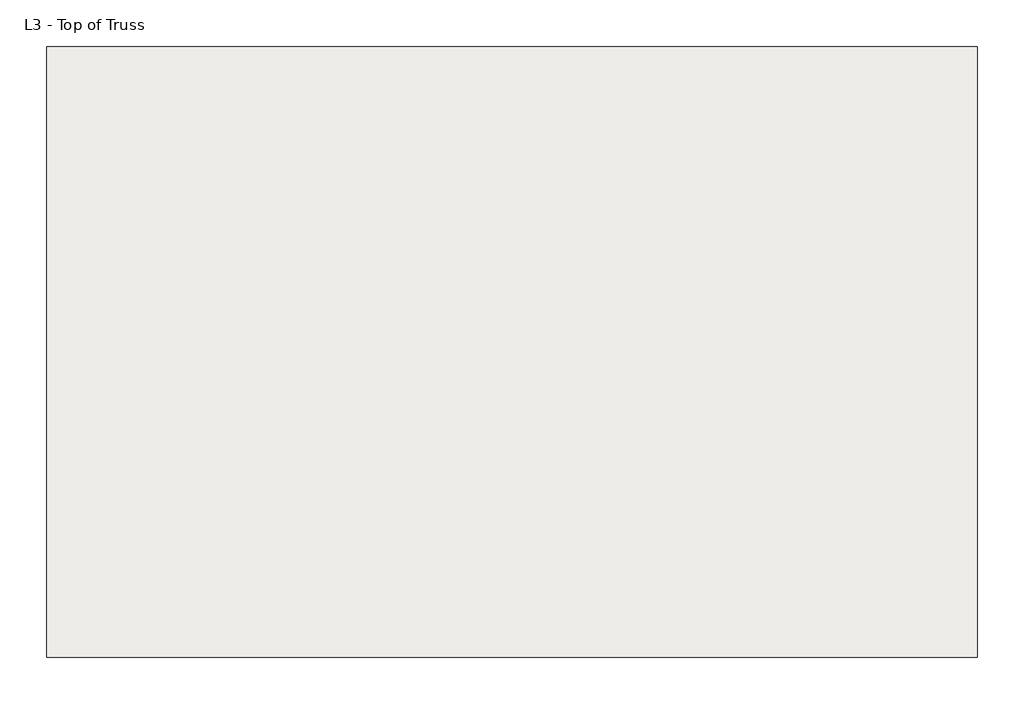
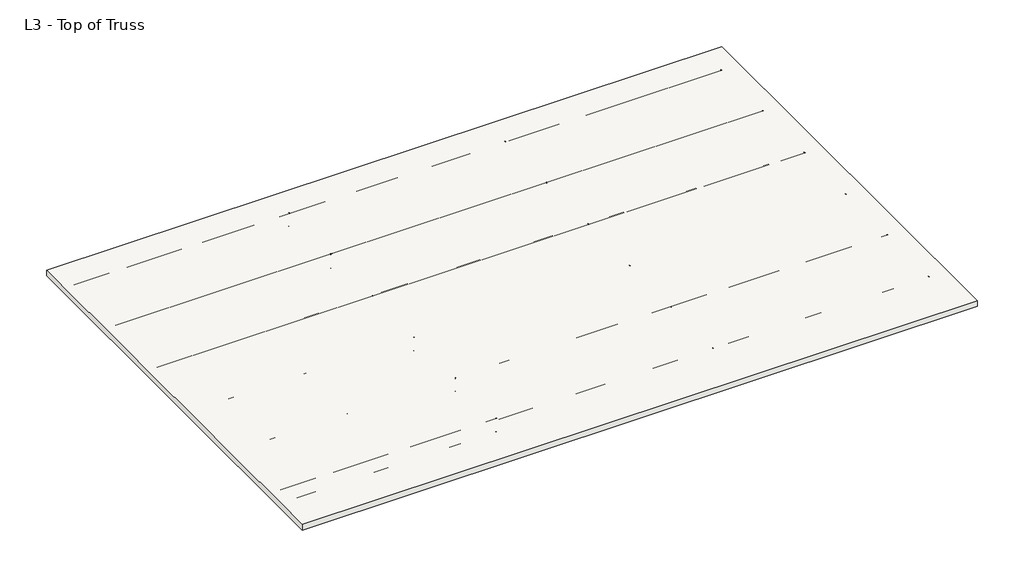
# One storey, part 1 of 2: 98 beams, 1 roof.
"""IFC4 building model written with IfcOpenShell, lengths in millimetres."""

import ifcopenshell
import ifcopenshell.guid

model = None  # the IFC model being written
_history = None  # IfcOwnerHistory: only IFC2X3 demands one
_inside = {}  # id of a spatial element -> (the spatial element, [elements in it])
_under = {}  # id of a project, library or spatial element -> (it, [spatial elements below it])
_declared = {}  # id of a project -> (the project, [libraries it declares])
_typed = {}  # id of a type object -> (the type object, [elements of that type])
_made_of = {}  # id of a material, layer set ... -> (it, [elements and type objects made of it])


def new_model(schema):
    """Start an empty IFC model of exactly this schema.

    Asked for "IFC4X3", IfcOpenShell would pick the latest addendum, in which some entities
    have other attributes; the version numbers below select the first issue.
    IFC2X3 requires an IfcOwnerHistory on every rooted entity: one is made here for all.
    """
    global model, _history
    if schema == "IFC4X3":
        model = ifcopenshell.file(schema_version=(4, 3, 0, 0))
    else:
        model = ifcopenshell.file(schema=schema)
    _inside.clear()
    _under.clear()
    _declared.clear()
    _typed.clear()
    _made_of.clear()
    _history = None
    if model.schema == "IFC2X3":
        org = make("IfcOrganization", Name="unknown")
        user = make(
            "IfcPersonAndOrganization",
            ThePerson=make("IfcPerson", FamilyName="unknown"),
            TheOrganization=org,
        )
        app = make(
            "IfcApplication",
            ApplicationDeveloper=org,
            Version="unknown",
            ApplicationFullName="unknown",
            ApplicationIdentifier="unknown",
        )
        _history = make(
            "IfcOwnerHistory",
            OwningUser=user,
            OwningApplication=app,
            ChangeAction="ADDED",
            CreationDate=0,
        )
    return model


def make(cls, **values):
    """One entity of the class cls with the attributes given. An attribute that is None is left unset."""
    return model.create_entity(
        cls, **{name: value for name, value in values.items() if value is not None}
    )


def rooted(cls, **values):
    """An entity with a GlobalId (a new one), such as an element, a storey or a relation."""
    return make(cls, GlobalId=ifcopenshell.guid.new(), OwnerHistory=_history, **values)


def si_unit(unit_type, name, prefix=None):
    """IfcSIUnit, for example si_unit("LENGTHUNIT", "METRE", prefix="MILLI")."""
    return make("IfcSIUnit", UnitType=unit_type, Prefix=prefix, Name=name)


def assignment(units):
    """IfcUnitAssignment: the units of a project."""
    return None if units is None else make("IfcUnitAssignment", Units=units)


def point(xyz):
    """IfcCartesianPoint."""
    return None if xyz is None else make("IfcCartesianPoint", Coordinates=xyz)


def direction(xyz):
    """IfcDirection."""
    return None if xyz is None else make("IfcDirection", DirectionRatios=xyz)


def frame(location, z_axis=None, x_axis=None):
    """IfcAxis2Placement3D, a coordinate frame: its origin and axes. An axis left out is left unset."""
    return make(
        "IfcAxis2Placement3D",
        Location=point(location),
        Axis=direction(z_axis),
        RefDirection=direction(x_axis),
    )


def frame_2d(location, x_axis=None):
    """IfcAxis2Placement2D, a coordinate frame in the plane: its origin and x axis."""
    return make(
        "IfcAxis2Placement2D", Location=point(location), RefDirection=direction(x_axis)
    )


def origin():
    """The frame at (0, 0, 0) with its axes left unset."""
    return frame((0.0, 0.0, 0.0))


def origin_2d():
    """The frame at (0, 0) in the plane with its x axis left unset."""
    return frame_2d((0.0, 0.0))


def place(relative_to, where):
    """IfcLocalPlacement: puts the frame where relative to a parent placement (None: the world)."""
    return make(
        "IfcLocalPlacement", PlacementRelTo=relative_to, RelativePlacement=where
    )


def context(
    kind, dimensions, precision=None, world=None, true_north=None, identifier=None
):
    """IfcGeometricRepresentationContext, for example the 3D "Model" context."""
    return make(
        "IfcGeometricRepresentationContext",
        ContextIdentifier=identifier,
        ContextType=kind,
        CoordinateSpaceDimension=dimensions,
        Precision=precision,
        WorldCoordinateSystem=world,
        TrueNorth=true_north,
    )


def project(units=None, contexts=None):
    """IfcProject with its units and contexts."""
    return rooted(
        "IfcProject",
        Name="project",
        RepresentationContexts=contexts,
        UnitsInContext=assignment(units),
    )


def spatial(cls, under=None, at=None, **own):
    """A site, building, storey or space (cls), placed at a placement, below another one or the project."""
    s = rooted(cls, ObjectPlacement=at, **own)
    if under is not None:
        _under.setdefault(under.id(), (under, []))[1].append(s)
    return s


def polyline(points):
    """IfcPolyline through the points."""
    return make("IfcPolyline", Points=[point(p) for p in points])


def circle_curve(where, radius):
    """IfcCircle in the frame where."""
    return make("IfcCircle", Position=where, Radius=radius)


def trimmed(basis, trim1, trim2, sense, master):
    """IfcTrimmedCurve: the piece of a basis curve between two trims."""
    return make(
        "IfcTrimmedCurve",
        BasisCurve=basis,
        Trim1=trim1,
        Trim2=trim2,
        SenseAgreement=sense,
        MasterRepresentation=master,
    )


def segment(curve, same_sense, transition):
    """IfcCompositeCurveSegment."""
    return make(
        "IfcCompositeCurveSegment",
        Transition=transition,
        SameSense=same_sense,
        ParentCurve=curve,
    )


def composite_curve(segments, self_intersect=None):
    """IfcCompositeCurve: segments joined end to end."""
    return make("IfcCompositeCurve", Segments=segments, SelfIntersect=self_intersect)


def outline(outer, holes=None, kind="AREA"):
    """IfcArbitraryClosedProfileDef: a profile drawn as a closed curve; with holes, ...WithVoids."""
    if holes is None:
        return make("IfcArbitraryClosedProfileDef", ProfileType=kind, OuterCurve=outer)
    return make(
        "IfcArbitraryProfileDefWithVoids",
        ProfileType=kind,
        OuterCurve=outer,
        InnerCurves=holes,
    )


def extrude(swept, where, along, depth):
    """IfcExtrudedAreaSolid: the profile swept, set in the frame where, extruded along a direction by depth."""
    return make(
        "IfcExtrudedAreaSolid",
        SweptArea=swept,
        Position=where,
        ExtrudedDirection=direction(along),
        Depth=depth,
    )


def shape(context_of_items, identifier, shape_type, items):
    """IfcShapeRepresentation: the items that make up one representation, for example the "Body"."""
    return make(
        "IfcShapeRepresentation",
        ContextOfItems=context_of_items,
        RepresentationIdentifier=identifier,
        RepresentationType=shape_type,
        Items=items,
    )


def source(mapping_origin, context_of_items, identifier, shape_type, items):
    """IfcRepresentationMap: a shape defined once, which mapped items show again and again."""
    return make(
        "IfcRepresentationMap",
        MappingOrigin=mapping_origin,
        MappedRepresentation=shape(context_of_items, identifier, shape_type, items),
    )


def transform(
    local_origin,
    x_axis=None,
    y_axis=None,
    z_axis=None,
    scale=None,
    scale2=None,
    scale3=None,
    uniform=True,
):
    """IfcCartesianTransformationOperator3D, or its non-uniform kind. x_axis, y_axis, z_axis: its Axis1, 2, 3."""
    if uniform:
        return make(
            "IfcCartesianTransformationOperator3D",
            Axis1=direction(x_axis),
            Axis2=direction(y_axis),
            LocalOrigin=point(local_origin),
            Scale=scale,
            Axis3=direction(z_axis),
        )
    return make(
        "IfcCartesianTransformationOperator3DnonUniform",
        Axis1=direction(x_axis),
        Axis2=direction(y_axis),
        LocalOrigin=point(local_origin),
        Scale=scale,
        Axis3=direction(z_axis),
        Scale2=scale2,
        Scale3=scale3,
    )


def mapped(mapping_source, mapping_target):
    """IfcMappedItem: shows the shape of a source again, moved by a transform."""
    return make(
        "IfcMappedItem", MappingSource=mapping_source, MappingTarget=mapping_target
    )


def made_of(thing, what):
    """Note that an element or type object is made of a material, layer set ...; save() writes the relation."""
    if what is not None:
        _made_of.setdefault(what.id(), (what, []))[1].append(thing)
    return thing


def element(
    cls,
    number,
    at=None,
    inside=None,
    cuts=None,
    type_object=None,
    material=None,
    context=None,
    identifier="Body",
    shape_type=None,
    held_by="IfcProductDefinitionShape",
    body=None,
    shapes=None,
    **own,
):
    """One element of the class cls, such as IfcWall. Its Tag is "e" and its number.

    at: its placement. inside: the storey or other place that contains it. cuts: it is an
    opening in that element (IfcRelVoidsElement). A single representation is given by context,
    identifier, shape_type and body (its items); several are given by shapes. held_by: the class
    of the entity that holds the representations. save() writes the other relations.
    """
    e = rooted(cls, Tag="e%d" % number, ObjectPlacement=at, **own)
    if body is not None:
        shapes = [shape(context, identifier, shape_type, body)]
    if shapes is not None:
        e.Representation = make(held_by, Representations=shapes)
    if inside is not None:
        _inside.setdefault(inside.id(), (inside, []))[1].append(e)
    if cuts is not None:
        rooted(
            "IfcRelVoidsElement", RelatingBuildingElement=cuts, RelatedOpeningElement=e
        )
    if type_object is not None:
        _typed.setdefault(type_object.id(), (type_object, []))[1].append(e)
    return made_of(e, material)


def aggregate(whole, parts):
    """IfcRelAggregates: a whole, such as a stair, and the parts it consists of."""
    return rooted("IfcRelAggregates", RelatingObject=whole, RelatedObjects=parts)


def save(model, path):
    """Write the relations noted so far, then the file.

    IfcRelAggregates (storeys below a building ...), IfcRelContainedInSpatialStructure (elements
    in a storey), IfcRelDefinesByType, IfcRelAssociatesMaterial and IfcRelDeclares: one each for
    every whole, place, type object, material and project.
    """
    for whole, parts in _under.values():
        aggregate(whole, parts)
    for where, things in _inside.values():
        rooted(
            "IfcRelContainedInSpatialStructure",
            RelatedElements=things,
            RelatingStructure=where,
        )
    for kind, things in _typed.values():
        rooted("IfcRelDefinesByType", RelatedObjects=things, RelatingType=kind)
    for what, things in _made_of.values():
        rooted("IfcRelAssociatesMaterial", RelatedObjects=things, RelatingMaterial=what)
    for by, libraries in _declared.values():
        rooted("IfcRelDeclares", RelatingContext=by, RelatedDefinitions=libraries)
    model.write(path)


def circular_hollow_sections_chs60_3x5_c94bd862(model_context):
    return source(origin(), model_context, "Body", "SweptSolid", [
        extrude(outline(composite_curve([segment(trimmed(circle_curve(origin_2d(), 30.15), [point((-30.15, 0.0))], [point((30.15, 0.0))], False, "CARTESIAN"), True, "CONTINUOUS"), segment(trimmed(circle_curve(origin_2d(), 30.15), [point((30.15, 0.0))], [point((-30.15, 0.0))], False, "CARTESIAN"), True, "CONTINUOUS")], self_intersect=False), holes=[composite_curve([segment(trimmed(circle_curve(origin_2d(), 25.15), [point((25.15, 0.0))], [point((-25.15, 0.0))], True, "CARTESIAN"), True, "CONTINUOUS"), segment(trimmed(circle_curve(origin_2d(), 25.15), [point((-25.15, 0.0))], [point((25.15, 0.0))], True, "CARTESIAN"), True, "CONTINUOUS")], self_intersect=False)]), frame((-557.0, 0.0, 0.0), z_axis=(1.0, 0.0, 0.0), x_axis=(0.0, 1.0, 0.0)), (0.0, 0.0, 1.0), 1114.0),
    ])


def circular_hollow_sections_chs60_3x5_b8a643cb(model_context):
    return source(origin(), model_context, "Body", "SweptSolid", [
        extrude(outline(composite_curve([segment(trimmed(circle_curve(origin_2d(), 30.15), [point((-30.15, 0.0))], [point((30.15, 0.0))], False, "CARTESIAN"), True, "CONTINUOUS"), segment(trimmed(circle_curve(origin_2d(), 30.15), [point((30.15, 0.0))], [point((-30.15, 0.0))], False, "CARTESIAN"), True, "CONTINUOUS")], self_intersect=False), holes=[composite_curve([segment(trimmed(circle_curve(origin_2d(), 25.15), [point((25.15, 0.0))], [point((-25.15, 0.0))], True, "CARTESIAN"), True, "CONTINUOUS"), segment(trimmed(circle_curve(origin_2d(), 25.15), [point((-25.15, 0.0))], [point((25.15, 0.0))], True, "CARTESIAN"), True, "CONTINUOUS")], self_intersect=False)]), frame((-790.0, 0.0, 0.0), z_axis=(1.0, 0.0, 0.0), x_axis=(0.0, 1.0, 0.0)), (0.0, 0.0, 1.0), 1580.0),
    ])


def circular_hollow_sections_chs60_3x5_ee2473de(model_context):
    return source(origin(), model_context, "Body", "SweptSolid", [
        extrude(outline(composite_curve([segment(trimmed(circle_curve(origin_2d(), 30.15), [point((-30.15, 0.0))], [point((30.15, 0.0))], False, "CARTESIAN"), True, "CONTINUOUS"), segment(trimmed(circle_curve(origin_2d(), 30.15), [point((30.15, 0.0))], [point((-30.15, 0.0))], False, "CARTESIAN"), True, "CONTINUOUS")], self_intersect=False), holes=[composite_curve([segment(trimmed(circle_curve(origin_2d(), 25.15), [point((25.15, 0.0))], [point((-25.15, 0.0))], True, "CARTESIAN"), True, "CONTINUOUS"), segment(trimmed(circle_curve(origin_2d(), 25.15), [point((-25.15, 0.0))], [point((25.15, 0.0))], True, "CARTESIAN"), True, "CONTINUOUS")], self_intersect=False)]), frame((-9000.0, 0.0, 0.0), z_axis=(1.0, 0.0, 0.0), x_axis=(0.0, 1.0, 0.0)), (0.0, 0.0, 1.0), 18000.0),
    ])


def circular_hollow_sections_chs60_3x5_7809bf4e(model_context):
    return source(origin(), model_context, "Body", "SweptSolid", [
        extrude(outline(composite_curve([segment(trimmed(circle_curve(origin_2d(), 30.15), [point((-30.15, 0.0))], [point((30.15, 0.0))], False, "CARTESIAN"), True, "CONTINUOUS"), segment(trimmed(circle_curve(origin_2d(), 30.15), [point((30.15, 0.0))], [point((-30.15, 0.0))], False, "CARTESIAN"), True, "CONTINUOUS")], self_intersect=False), holes=[composite_curve([segment(trimmed(circle_curve(origin_2d(), 25.15), [point((25.15, 0.0))], [point((-25.15, 0.0))], True, "CARTESIAN"), True, "CONTINUOUS"), segment(trimmed(circle_curve(origin_2d(), 25.15), [point((-25.15, 0.0))], [point((25.15, 0.0))], True, "CARTESIAN"), True, "CONTINUOUS")], self_intersect=False)]), frame((-600.0, 0.0, 0.0), z_axis=(1.0, 0.0, 0.0), x_axis=(0.0, 1.0, 0.0)), (0.0, 0.0, 1.0), 1157.0),
    ])


model = new_model("IFC4")

# Units and contexts
model_context = context("Model", 3, world=origin())
ifc_project = project(units=[si_unit("LENGTHUNIT", "METRE", prefix="MILLI")], contexts=[model_context])

# Site, building, storey
site = spatial("IfcSite", under=ifc_project)
building = spatial("IfcBuilding", under=site)
storey = spatial("IfcBuildingStorey", under=building, Name="L3 - Top of Truss", Elevation=7800.0)

# Beams
placement = place(None, origin())
circular_hollow_sections_chs60_3x5_shape = circular_hollow_sections_chs60_3x5_c94bd862(model_context)
element("IfcBeam", 1, ObjectType="Circular Hollow Sections : CHS60.3x5", at=placement, inside=storey, context=model_context, shape_type="MappedRepresentation", body=[
    mapped(circular_hollow_sections_chs60_3x5_shape, transform((-5853.84106, -5058.7619082, 7200.0), x_axis=(0.0, 0.0, 1.0), y_axis=(0.0, -1.0, 0.0), z_axis=(1.0, 0.0, 0.0))),
])
element("IfcBeam", 2, ObjectType="Circular Hollow Sections : CHS60.3x5", at=placement, inside=storey, context=model_context, shape_type="MappedRepresentation", body=[
    mapped(circular_hollow_sections_chs60_3x5_shape, transform((-4568.1267743, -5058.7619082, 7200.0), x_axis=(0.0, 0.0, 1.0), y_axis=(0.0, -1.0, 0.0), z_axis=(1.0, 0.0, 0.0))),
])
element("IfcBeam", 3, ObjectType="Circular Hollow Sections : CHS60.3x5", at=placement, inside=storey, context=model_context, shape_type="MappedRepresentation", body=[
    mapped(circular_hollow_sections_chs60_3x5_shape, transform((-3282.4124885, -5058.7619082, 7200.0), x_axis=(0.0, 0.0, 1.0), y_axis=(0.0, -1.0, 0.0), z_axis=(1.0, 0.0, 0.0))),
])
element("IfcBeam", 4, ObjectType="Circular Hollow Sections : CHS60.3x5", at=placement, inside=storey, context=model_context, shape_type="MappedRepresentation", body=[
    mapped(circular_hollow_sections_chs60_3x5_shape, transform((-1996.6982028, -5058.7619082, 7200.0), x_axis=(0.0, 0.0, 1.0), y_axis=(0.0, -1.0, 0.0), z_axis=(1.0, 0.0, 0.0))),
])
element("IfcBeam", 5, ObjectType="Circular Hollow Sections : CHS60.3x5", at=placement, inside=storey, context=model_context, shape_type="MappedRepresentation", body=[
    mapped(circular_hollow_sections_chs60_3x5_shape, transform((-710.9839171, -5058.7619082, 7200.0), x_axis=(0.0, 0.0, 1.0), y_axis=(0.0, -1.0, 0.0), z_axis=(1.0, 0.0, 0.0))),
])
element("IfcBeam", 6, ObjectType="Circular Hollow Sections : CHS60.3x5", at=placement, inside=storey, context=model_context, shape_type="MappedRepresentation", body=[
    mapped(circular_hollow_sections_chs60_3x5_shape, transform((-5853.84106, -11058.7619082, 7200.0), x_axis=(0.0, 0.0, 1.0), y_axis=(0.0, -1.0, 0.0), z_axis=(1.0, 0.0, 0.0))),
])
element("IfcBeam", 7, ObjectType="Circular Hollow Sections : CHS60.3x5", at=placement, inside=storey, context=model_context, shape_type="MappedRepresentation", body=[
    mapped(circular_hollow_sections_chs60_3x5_shape, transform((-4568.1267743, -11058.7619082, 7200.0), x_axis=(0.0, 0.0, 1.0), y_axis=(0.0, -1.0, 0.0), z_axis=(1.0, 0.0, 0.0))),
])
element("IfcBeam", 8, ObjectType="Circular Hollow Sections : CHS60.3x5", at=placement, inside=storey, context=model_context, shape_type="MappedRepresentation", body=[
    mapped(circular_hollow_sections_chs60_3x5_shape, transform((-3282.4124885, -11058.7619082, 7200.0), x_axis=(0.0, 0.0, 1.0), y_axis=(0.0, -1.0, 0.0), z_axis=(1.0, 0.0, 0.0))),
])
element("IfcBeam", 9, ObjectType="Circular Hollow Sections : CHS60.3x5", at=placement, inside=storey, context=model_context, shape_type="MappedRepresentation", body=[
    mapped(circular_hollow_sections_chs60_3x5_shape, transform((5717.5875115, -11058.7619082, 7200.0), x_axis=(0.0, 0.0, 1.0), y_axis=(0.0, -1.0, 0.0), z_axis=(1.0, 0.0, 0.0))),
])
element("IfcBeam", 10, ObjectType="Circular Hollow Sections : CHS60.3x5", at=placement, inside=storey, context=model_context, shape_type="MappedRepresentation", body=[
    mapped(circular_hollow_sections_chs60_3x5_shape, transform((4431.8732257, -11058.7619082, 7200.0), x_axis=(0.0, 0.0, 1.0), y_axis=(0.0, -1.0, 0.0), z_axis=(1.0, 0.0, 0.0))),
])
element("IfcBeam", 11, ObjectType="Circular Hollow Sections : CHS60.3x5", at=placement, inside=storey, context=model_context, shape_type="MappedRepresentation", body=[
    mapped(circular_hollow_sections_chs60_3x5_shape, transform((3146.15894, -11058.7619082, 7200.0), x_axis=(0.0, 0.0, 1.0), y_axis=(0.0, -1.0, 0.0), z_axis=(1.0, 0.0, 0.0))),
])
element("IfcBeam", 12, ObjectType="Circular Hollow Sections : CHS60.3x5", at=placement, inside=storey, context=model_context, shape_type="MappedRepresentation", body=[
    mapped(circular_hollow_sections_chs60_3x5_shape, transform((-1996.6982028, -11058.7619082, 7200.0), x_axis=(0.0, 0.0, 1.0), y_axis=(0.0, -1.0, 0.0), z_axis=(1.0, 0.0, 0.0))),
])
element("IfcBeam", 13, ObjectType="Circular Hollow Sections : CHS60.3x5", at=placement, inside=storey, context=model_context, shape_type="MappedRepresentation", body=[
    mapped(circular_hollow_sections_chs60_3x5_shape, transform((-710.9839171, -11058.7619082, 7200.0), x_axis=(0.0, 0.0, 1.0), y_axis=(0.0, -1.0, 0.0), z_axis=(1.0, 0.0, 0.0))),
])
element("IfcBeam", 14, ObjectType="Circular Hollow Sections : CHS60.3x5", at=placement, inside=storey, context=model_context, shape_type="MappedRepresentation", body=[
    mapped(circular_hollow_sections_chs60_3x5_shape, transform((574.7303686, -11058.7619082, 7200.0), x_axis=(0.0, 0.0, 1.0), y_axis=(0.0, -1.0, 0.0), z_axis=(1.0, 0.0, 0.0))),
])
element("IfcBeam", 15, ObjectType="Circular Hollow Sections : CHS60.3x5", at=placement, inside=storey, context=model_context, shape_type="MappedRepresentation", body=[
    mapped(circular_hollow_sections_chs60_3x5_shape, transform((1860.4446543, -11058.7619082, 7200.0), x_axis=(0.0, 0.0, 1.0), y_axis=(0.0, -1.0, 0.0), z_axis=(1.0, 0.0, 0.0))),
])
element("IfcBeam", 16, ObjectType="Circular Hollow Sections : CHS60.3x5", at=placement, inside=storey, context=model_context, shape_type="MappedRepresentation", body=[
    mapped(circular_hollow_sections_chs60_3x5_shape, transform((9574.7303686, -17058.7619082, 7200.0), x_axis=(0.0, 0.0, 1.0), y_axis=(0.0, -1.0, 0.0), z_axis=(1.0, 0.0, 0.0))),
])
element("IfcBeam", 17, ObjectType="Circular Hollow Sections : CHS60.3x5", at=placement, inside=storey, context=model_context, shape_type="MappedRepresentation", body=[
    mapped(circular_hollow_sections_chs60_3x5_shape, transform((-5853.84106, -17058.7619082, 7200.0), x_axis=(0.0, 0.0, 1.0), y_axis=(0.0, -1.0, 0.0), z_axis=(1.0, 0.0, 0.0))),
])
element("IfcBeam", 18, ObjectType="Circular Hollow Sections : CHS60.3x5", at=placement, inside=storey, context=model_context, shape_type="MappedRepresentation", body=[
    mapped(circular_hollow_sections_chs60_3x5_shape, transform((8289.0160829, -17058.7619082, 7200.0), x_axis=(0.0, 0.0, 1.0), y_axis=(0.0, -1.0, 0.0), z_axis=(1.0, 0.0, 0.0))),
])
element("IfcBeam", 19, ObjectType="Circular Hollow Sections : CHS60.3x5", at=placement, inside=storey, context=model_context, shape_type="MappedRepresentation", body=[
    mapped(circular_hollow_sections_chs60_3x5_shape, transform((-4568.1267743, -17058.7619082, 7200.0), x_axis=(0.0, 0.0, 1.0), y_axis=(0.0, -1.0, 0.0), z_axis=(1.0, 0.0, 0.0))),
])
element("IfcBeam", 20, ObjectType="Circular Hollow Sections : CHS60.3x5", at=placement, inside=storey, context=model_context, shape_type="MappedRepresentation", body=[
    mapped(circular_hollow_sections_chs60_3x5_shape, transform((7003.3017972, -17058.7619082, 7200.0), x_axis=(0.0, 0.0, 1.0), y_axis=(0.0, -1.0, 0.0), z_axis=(1.0, 0.0, 0.0))),
])
element("IfcBeam", 21, ObjectType="Circular Hollow Sections : CHS60.3x5", at=placement, inside=storey, context=model_context, shape_type="MappedRepresentation", body=[
    mapped(circular_hollow_sections_chs60_3x5_shape, transform((-3282.4124885, -17058.7619082, 7200.0), x_axis=(0.0, 0.0, 1.0), y_axis=(0.0, -1.0, 0.0), z_axis=(1.0, 0.0, 0.0))),
])
element("IfcBeam", 22, ObjectType="Circular Hollow Sections : CHS60.3x5", at=placement, inside=storey, context=model_context, shape_type="MappedRepresentation", body=[
    mapped(circular_hollow_sections_chs60_3x5_shape, transform((5717.5875115, -17058.7619082, 7200.0), x_axis=(0.0, 0.0, 1.0), y_axis=(0.0, -1.0, 0.0), z_axis=(1.0, 0.0, 0.0))),
])
element("IfcBeam", 23, ObjectType="Circular Hollow Sections : CHS60.3x5", at=placement, inside=storey, context=model_context, shape_type="MappedRepresentation", body=[
    mapped(circular_hollow_sections_chs60_3x5_shape, transform((4431.8732257, -17058.7619082, 7200.0), x_axis=(0.0, 0.0, 1.0), y_axis=(0.0, -1.0, 0.0), z_axis=(1.0, 0.0, 0.0))),
])
element("IfcBeam", 24, ObjectType="Circular Hollow Sections : CHS60.3x5", at=placement, inside=storey, context=model_context, shape_type="MappedRepresentation", body=[
    mapped(circular_hollow_sections_chs60_3x5_shape, transform((3146.15894, -17058.7619082, 7200.0), x_axis=(0.0, 0.0, 1.0), y_axis=(0.0, -1.0, 0.0), z_axis=(1.0, 0.0, 0.0))),
])
element("IfcBeam", 25, ObjectType="Circular Hollow Sections : CHS60.3x5", at=placement, inside=storey, context=model_context, shape_type="MappedRepresentation", body=[
    mapped(circular_hollow_sections_chs60_3x5_shape, transform((-1996.6982028, -17058.7619082, 7200.0), x_axis=(0.0, 0.0, 1.0), y_axis=(0.0, -1.0, 0.0), z_axis=(1.0, 0.0, 0.0))),
])
element("IfcBeam", 26, ObjectType="Circular Hollow Sections : CHS60.3x5", at=placement, inside=storey, context=model_context, shape_type="MappedRepresentation", body=[
    mapped(circular_hollow_sections_chs60_3x5_shape, transform((-710.9839171, -17058.7619082, 7200.0), x_axis=(0.0, 0.0, 1.0), y_axis=(0.0, -1.0, 0.0), z_axis=(1.0, 0.0, 0.0))),
])
element("IfcBeam", 27, ObjectType="Circular Hollow Sections : CHS60.3x5", at=placement, inside=storey, context=model_context, shape_type="MappedRepresentation", body=[
    mapped(circular_hollow_sections_chs60_3x5_shape, transform((574.7303686, -17058.7619082, 7200.0), x_axis=(0.0, 0.0, 1.0), y_axis=(0.0, -1.0, 0.0), z_axis=(1.0, 0.0, 0.0))),
])
element("IfcBeam", 28, ObjectType="Circular Hollow Sections : CHS60.3x5", at=placement, inside=storey, context=model_context, shape_type="MappedRepresentation", body=[
    mapped(circular_hollow_sections_chs60_3x5_shape, transform((1860.4446543, -17058.7619082, 7200.0), x_axis=(0.0, 0.0, 1.0), y_axis=(0.0, -1.0, 0.0), z_axis=(1.0, 0.0, 0.0))),
])
element("IfcBeam", 29, ObjectType="Circular Hollow Sections : CHS60.3x5", at=placement, inside=storey, context=model_context, shape_type="MappedRepresentation", body=[
    mapped(circular_hollow_sections_chs60_3x5_shape, transform((9574.7303686, -22948.7619082, 7200.0), x_axis=(0.0, 0.0, 1.0), y_axis=(0.0, -1.0, 0.0), z_axis=(1.0, 0.0, 0.0))),
])
element("IfcBeam", 30, ObjectType="Circular Hollow Sections : CHS60.3x5", at=placement, inside=storey, context=model_context, shape_type="MappedRepresentation", body=[
    mapped(circular_hollow_sections_chs60_3x5_shape, transform((-5853.84106, -22948.7619082, 7200.0), x_axis=(0.0, 0.0, 1.0), y_axis=(0.0, -1.0, 0.0), z_axis=(1.0, 0.0, 0.0))),
])
element("IfcBeam", 31, ObjectType="Circular Hollow Sections : CHS60.3x5", at=placement, inside=storey, context=model_context, shape_type="MappedRepresentation", body=[
    mapped(circular_hollow_sections_chs60_3x5_shape, transform((8289.0160829, -22948.7619082, 7200.0), x_axis=(0.0, 0.0, 1.0), y_axis=(0.0, -1.0, 0.0), z_axis=(1.0, 0.0, 0.0))),
])
element("IfcBeam", 32, ObjectType="Circular Hollow Sections : CHS60.3x5", at=placement, inside=storey, context=model_context, shape_type="MappedRepresentation", body=[
    mapped(circular_hollow_sections_chs60_3x5_shape, transform((-4568.1267743, -22948.7619082, 7200.0), x_axis=(0.0, 0.0, 1.0), y_axis=(0.0, -1.0, 0.0), z_axis=(1.0, 0.0, 0.0))),
])
element("IfcBeam", 33, ObjectType="Circular Hollow Sections : CHS60.3x5", at=placement, inside=storey, context=model_context, shape_type="MappedRepresentation", body=[
    mapped(circular_hollow_sections_chs60_3x5_shape, transform((7003.3017972, -22948.7619082, 7200.0), x_axis=(0.0, 0.0, 1.0), y_axis=(0.0, -1.0, 0.0), z_axis=(1.0, 0.0, 0.0))),
])
element("IfcBeam", 34, ObjectType="Circular Hollow Sections : CHS60.3x5", at=placement, inside=storey, context=model_context, shape_type="MappedRepresentation", body=[
    mapped(circular_hollow_sections_chs60_3x5_shape, transform((-3282.4124885, -22948.7619082, 7200.0), x_axis=(0.0, 0.0, 1.0), y_axis=(0.0, -1.0, 0.0), z_axis=(1.0, 0.0, 0.0))),
])
element("IfcBeam", 35, ObjectType="Circular Hollow Sections : CHS60.3x5", at=placement, inside=storey, context=model_context, shape_type="MappedRepresentation", body=[
    mapped(circular_hollow_sections_chs60_3x5_shape, transform((5717.5875115, -22948.7619082, 7200.0), x_axis=(0.0, 0.0, 1.0), y_axis=(0.0, -1.0, 0.0), z_axis=(1.0, 0.0, 0.0))),
])
element("IfcBeam", 36, ObjectType="Circular Hollow Sections : CHS60.3x5", at=placement, inside=storey, context=model_context, shape_type="MappedRepresentation", body=[
    mapped(circular_hollow_sections_chs60_3x5_shape, transform((4431.8732257, -22948.7619082, 7200.0), x_axis=(0.0, 0.0, 1.0), y_axis=(0.0, -1.0, 0.0), z_axis=(1.0, 0.0, 0.0))),
])
element("IfcBeam", 37, ObjectType="Circular Hollow Sections : CHS60.3x5", at=placement, inside=storey, context=model_context, shape_type="MappedRepresentation", body=[
    mapped(circular_hollow_sections_chs60_3x5_shape, transform((10860.4446543, -22948.7619082, 7200.0), x_axis=(0.0, 0.0, 1.0), y_axis=(0.0, -1.0, 0.0), z_axis=(1.0, 0.0, 0.0))),
])
element("IfcBeam", 38, ObjectType="Circular Hollow Sections : CHS60.3x5", at=placement, inside=storey, context=model_context, shape_type="MappedRepresentation", body=[
    mapped(circular_hollow_sections_chs60_3x5_shape, transform((3146.15894, -22948.7619082, 7200.0), x_axis=(0.0, 0.0, 1.0), y_axis=(0.0, -1.0, 0.0), z_axis=(1.0, 0.0, 0.0))),
])
element("IfcBeam", 39, ObjectType="Circular Hollow Sections : CHS60.3x5", at=placement, inside=storey, context=model_context, shape_type="MappedRepresentation", body=[
    mapped(circular_hollow_sections_chs60_3x5_shape, transform((-1996.6982028, -22948.7619082, 7200.0), x_axis=(0.0, 0.0, 1.0), y_axis=(0.0, -1.0, 0.0), z_axis=(1.0, 0.0, 0.0))),
])
element("IfcBeam", 40, ObjectType="Circular Hollow Sections : CHS60.3x5", at=placement, inside=storey, context=model_context, shape_type="MappedRepresentation", body=[
    mapped(circular_hollow_sections_chs60_3x5_shape, transform((-710.9839171, -22948.7619082, 7200.0), x_axis=(0.0, 0.0, 1.0), y_axis=(0.0, -1.0, 0.0), z_axis=(1.0, 0.0, 0.0))),
])
element("IfcBeam", 41, ObjectType="Circular Hollow Sections : CHS60.3x5", at=placement, inside=storey, context=model_context, shape_type="MappedRepresentation", body=[
    mapped(circular_hollow_sections_chs60_3x5_shape, transform((-7139.5553457, -22948.7619082, 7200.0), x_axis=(0.0, 0.0, 1.0), y_axis=(0.0, -1.0, 0.0), z_axis=(1.0, 0.0, 0.0))),
])
element("IfcBeam", 42, ObjectType="Circular Hollow Sections : CHS60.3x5", at=placement, inside=storey, context=model_context, shape_type="MappedRepresentation", body=[
    mapped(circular_hollow_sections_chs60_3x5_shape, transform((574.7303686, -22948.7619082, 7200.0), x_axis=(0.0, 0.0, 1.0), y_axis=(0.0, -1.0, 0.0), z_axis=(1.0, 0.0, 0.0))),
])
element("IfcBeam", 43, ObjectType="Circular Hollow Sections : CHS60.3x5", at=placement, inside=storey, context=model_context, shape_type="MappedRepresentation", body=[
    mapped(circular_hollow_sections_chs60_3x5_shape, transform((1860.4446543, -22948.7619082, 7200.0), x_axis=(0.0, 0.0, 1.0), y_axis=(0.0, -1.0, 0.0), z_axis=(1.0, 0.0, 0.0))),
])
circular_hollow_sections_chs60_3x5_2_shape = circular_hollow_sections_chs60_3x5_b8a643cb(model_context)
element("IfcBeam", 44, ObjectType="Circular Hollow Sections : CHS60.3x5", at=placement, inside=storey, context=model_context, shape_type="MappedRepresentation", body=[
    mapped(circular_hollow_sections_chs60_3x5_2_shape, transform((-5210.9839171, -5058.7619082, 7200.0), x_axis=(0.7310552682428689, 0.0, -0.6823182503600113), y_axis=(0.0, -1.0, 0.0), z_axis=(-0.6823182503600113, 0.0, -0.7310552682428689))),
])
element("IfcBeam", 45, ObjectType="Circular Hollow Sections : CHS60.3x5", at=placement, inside=storey, context=model_context, shape_type="MappedRepresentation", body=[
    mapped(circular_hollow_sections_chs60_3x5_2_shape, transform((-3925.2696314, -5058.7619082, 7200.0), x_axis=(0.7310552682428689, 0.0, -0.6823182503600113), y_axis=(0.0, -1.0, 0.0), z_axis=(-0.6823182503600113, 0.0, -0.7310552682428689))),
])
element("IfcBeam", 46, ObjectType="Circular Hollow Sections : CHS60.3x5", at=placement, inside=storey, context=model_context, shape_type="MappedRepresentation", body=[
    mapped(circular_hollow_sections_chs60_3x5_2_shape, transform((-2639.5553457, -5058.7619082, 7200.0), x_axis=(0.7310552682428689, 0.0, -0.6823182503600113), y_axis=(0.0, -1.0, 0.0), z_axis=(-0.6823182503600113, 0.0, -0.7310552682428689))),
])
element("IfcBeam", 47, ObjectType="Circular Hollow Sections : CHS60.3x5", at=placement, inside=storey, context=model_context, shape_type="MappedRepresentation", body=[
    mapped(circular_hollow_sections_chs60_3x5_2_shape, transform((-1353.84106, -5058.7619082, 7200.0), x_axis=(0.7310552682428689, 0.0, -0.6823182503600113), y_axis=(0.0, -1.0, 0.0), z_axis=(-0.6823182503600113, 0.0, -0.7310552682428689))),
])
element("IfcBeam", 48, ObjectType="Circular Hollow Sections : CHS60.3x5", at=placement, inside=storey, context=model_context, shape_type="MappedRepresentation", body=[
    mapped(circular_hollow_sections_chs60_3x5_2_shape, transform((-68.1267743, -5058.7619082, 7200.0), x_axis=(0.7310552682428689, 0.0, -0.6823182503600113), y_axis=(0.0, -1.0, 0.0), z_axis=(-0.6823182503600113, 0.0, -0.7310552682428689))),
])
element("IfcBeam", 49, ObjectType="Circular Hollow Sections : CHS60.3x5", at=placement, inside=storey, context=model_context, shape_type="MappedRepresentation", body=[
    mapped(circular_hollow_sections_chs60_3x5_2_shape, transform((-6496.6982028, -5058.7619082, 7200.0), x_axis=(0.7310552682428691, 0.0, -0.6823182503600111), y_axis=(0.0, -1.0, 0.0), z_axis=(-0.6823182503600111, 0.0, -0.7310552682428691))),
])
element("IfcBeam", 50, ObjectType="Circular Hollow Sections : CHS60.3x5", at=placement, inside=storey, context=model_context, shape_type="MappedRepresentation", body=[
    mapped(circular_hollow_sections_chs60_3x5_2_shape, transform((-5210.9839171, -11058.7619082, 7200.0), x_axis=(0.7310552682428689, 0.0, -0.6823182503600113), y_axis=(0.0, -1.0, 0.0), z_axis=(-0.6823182503600113, 0.0, -0.7310552682428689))),
])
element("IfcBeam", 51, ObjectType="Circular Hollow Sections : CHS60.3x5", at=placement, inside=storey, context=model_context, shape_type="MappedRepresentation", body=[
    mapped(circular_hollow_sections_chs60_3x5_2_shape, transform((-3925.2696314, -11058.7619082, 7200.0), x_axis=(0.7310552682428689, 0.0, -0.6823182503600113), y_axis=(0.0, -1.0, 0.0), z_axis=(-0.6823182503600113, 0.0, -0.7310552682428689))),
])
element("IfcBeam", 52, ObjectType="Circular Hollow Sections : CHS60.3x5", at=placement, inside=storey, context=model_context, shape_type="MappedRepresentation", body=[
    mapped(circular_hollow_sections_chs60_3x5_2_shape, transform((-2639.5553457, -11058.7619082, 7200.0), x_axis=(0.7310552682428689, 0.0, -0.6823182503600113), y_axis=(0.0, -1.0, 0.0), z_axis=(-0.6823182503600113, 0.0, -0.7310552682428689))),
])
element("IfcBeam", 53, ObjectType="Circular Hollow Sections : CHS60.3x5", at=placement, inside=storey, context=model_context, shape_type="MappedRepresentation", body=[
    mapped(circular_hollow_sections_chs60_3x5_2_shape, transform((3789.0160829, -11058.7619082, 7200.0), x_axis=(0.7310552682428691, 0.0, 0.6823182503600111), y_axis=(0.0, -1.0, 0.0), z_axis=(0.6823182503600111, 0.0, -0.7310552682428691))),
])
element("IfcBeam", 54, ObjectType="Circular Hollow Sections : CHS60.3x5", at=placement, inside=storey, context=model_context, shape_type="MappedRepresentation", body=[
    mapped(circular_hollow_sections_chs60_3x5_2_shape, transform((2503.3017972, -11058.7619082, 7200.0), x_axis=(0.7310552682428691, 0.0, 0.682318250360011), y_axis=(0.0, -1.0, 0.0), z_axis=(0.682318250360011, 0.0, -0.7310552682428691))),
])
element("IfcBeam", 55, ObjectType="Circular Hollow Sections : CHS60.3x5", at=placement, inside=storey, context=model_context, shape_type="MappedRepresentation", body=[
    mapped(circular_hollow_sections_chs60_3x5_2_shape, transform((-1353.84106, -11058.7619082, 7200.0), x_axis=(0.7310552682428689, 0.0, -0.6823182503600113), y_axis=(0.0, -1.0, 0.0), z_axis=(-0.6823182503600113, 0.0, -0.7310552682428689))),
])
element("IfcBeam", 56, ObjectType="Circular Hollow Sections : CHS60.3x5", at=placement, inside=storey, context=model_context, shape_type="MappedRepresentation", body=[
    mapped(circular_hollow_sections_chs60_3x5_2_shape, transform((-68.1267743, -11058.7619082, 7200.0), x_axis=(0.7310552682428689, 0.0, -0.6823182503600113), y_axis=(0.0, -1.0, 0.0), z_axis=(-0.6823182503600113, 0.0, -0.7310552682428689))),
])
element("IfcBeam", 57, ObjectType="Circular Hollow Sections : CHS60.3x5", at=placement, inside=storey, context=model_context, shape_type="MappedRepresentation", body=[
    mapped(circular_hollow_sections_chs60_3x5_2_shape, transform((-6496.6982028, -11058.7619082, 7200.0), x_axis=(0.7310552682428688, 0.0, -0.6823182503600115), y_axis=(0.0, -1.0, 0.0), z_axis=(-0.6823182503600115, 0.0, -0.7310552682428688))),
])
element("IfcBeam", 58, ObjectType="Circular Hollow Sections : CHS60.3x5", at=placement, inside=storey, context=model_context, shape_type="MappedRepresentation", body=[
    mapped(circular_hollow_sections_chs60_3x5_2_shape, transform((1217.5875115, -11058.7619082, 7200.0), x_axis=(0.7310552682428689, 0.0, -0.6823182503600113), y_axis=(0.0, -1.0, 0.0), z_axis=(-0.6823182503600113, 0.0, -0.7310552682428689))),
])
element("IfcBeam", 59, ObjectType="Circular Hollow Sections : CHS60.3x5", at=placement, inside=storey, context=model_context, shape_type="MappedRepresentation", body=[
    mapped(circular_hollow_sections_chs60_3x5_2_shape, transform((8931.8732257, -17058.7619082, 7200.0), x_axis=(0.7310552682428691, 0.0, 0.6823182503600111), y_axis=(0.0, -1.0, 0.0), z_axis=(0.6823182503600111, 0.0, -0.7310552682428691))),
])
element("IfcBeam", 60, ObjectType="Circular Hollow Sections : CHS60.3x5", at=placement, inside=storey, context=model_context, shape_type="MappedRepresentation", body=[
    mapped(circular_hollow_sections_chs60_3x5_2_shape, transform((-5210.9839171, -17058.7619082, 7200.0), x_axis=(0.7310552682428689, 0.0, -0.6823182503600113), y_axis=(0.0, -1.0, 0.0), z_axis=(-0.6823182503600113, 0.0, -0.7310552682428689))),
])
element("IfcBeam", 61, ObjectType="Circular Hollow Sections : CHS60.3x5", at=placement, inside=storey, context=model_context, shape_type="MappedRepresentation", body=[
    mapped(circular_hollow_sections_chs60_3x5_2_shape, transform((7646.15894, -17058.7619082, 7200.0), x_axis=(0.7310552682428691, 0.0, 0.6823182503600111), y_axis=(0.0, -1.0, 0.0), z_axis=(0.6823182503600111, 0.0, -0.7310552682428691))),
])
element("IfcBeam", 62, ObjectType="Circular Hollow Sections : CHS60.3x5", at=placement, inside=storey, context=model_context, shape_type="MappedRepresentation", body=[
    mapped(circular_hollow_sections_chs60_3x5_2_shape, transform((-3925.2696314, -17058.7619082, 7200.0), x_axis=(0.7310552682428689, 0.0, -0.6823182503600113), y_axis=(0.0, -1.0, 0.0), z_axis=(-0.6823182503600113, 0.0, -0.7310552682428689))),
])
element("IfcBeam", 63, ObjectType="Circular Hollow Sections : CHS60.3x5", at=placement, inside=storey, context=model_context, shape_type="MappedRepresentation", body=[
    mapped(circular_hollow_sections_chs60_3x5_2_shape, transform((6360.4446543, -17058.7619082, 7200.0), x_axis=(0.7310552682428691, 0.0, 0.6823182503600111), y_axis=(0.0, -1.0, 0.0), z_axis=(0.6823182503600111, 0.0, -0.7310552682428691))),
])
element("IfcBeam", 64, ObjectType="Circular Hollow Sections : CHS60.3x5", at=placement, inside=storey, context=model_context, shape_type="MappedRepresentation", body=[
    mapped(circular_hollow_sections_chs60_3x5_2_shape, transform((-2639.5553457, -17058.7619082, 7200.0), x_axis=(0.7310552682428689, 0.0, -0.6823182503600113), y_axis=(0.0, -1.0, 0.0), z_axis=(-0.6823182503600113, 0.0, -0.7310552682428689))),
])
element("IfcBeam", 65, ObjectType="Circular Hollow Sections : CHS60.3x5", at=placement, inside=storey, context=model_context, shape_type="MappedRepresentation", body=[
    mapped(circular_hollow_sections_chs60_3x5_2_shape, transform((5074.7303686, -17058.7619082, 7200.0), x_axis=(0.7310552682428691, 0.0, 0.6823182503600111), y_axis=(0.0, -1.0, 0.0), z_axis=(0.6823182503600111, 0.0, -0.7310552682428691))),
])
element("IfcBeam", 66, ObjectType="Circular Hollow Sections : CHS60.3x5", at=placement, inside=storey, context=model_context, shape_type="MappedRepresentation", body=[
    mapped(circular_hollow_sections_chs60_3x5_2_shape, transform((3789.0160829, -17058.7619082, 7200.0), x_axis=(0.7310552682428691, 0.0, 0.6823182503600111), y_axis=(0.0, -1.0, 0.0), z_axis=(0.6823182503600111, 0.0, -0.7310552682428691))),
])
element("IfcBeam", 67, ObjectType="Circular Hollow Sections : CHS60.3x5", at=placement, inside=storey, context=model_context, shape_type="MappedRepresentation", body=[
    mapped(circular_hollow_sections_chs60_3x5_2_shape, transform((10217.5875115, -17058.7619082, 7200.0), x_axis=(0.7310552682428691, 0.0, 0.6823182503600111), y_axis=(0.0, -1.0, 0.0), z_axis=(0.6823182503600111, 0.0, -0.7310552682428691))),
])
element("IfcBeam", 68, ObjectType="Circular Hollow Sections : CHS60.3x5", at=placement, inside=storey, context=model_context, shape_type="MappedRepresentation", body=[
    mapped(circular_hollow_sections_chs60_3x5_2_shape, transform((2503.3017972, -17058.7619082, 7200.0), x_axis=(0.7310552682428691, 0.0, 0.682318250360011), y_axis=(0.0, -1.0, 0.0), z_axis=(0.682318250360011, 0.0, -0.7310552682428691))),
])
element("IfcBeam", 69, ObjectType="Circular Hollow Sections : CHS60.3x5", at=placement, inside=storey, context=model_context, shape_type="MappedRepresentation", body=[
    mapped(circular_hollow_sections_chs60_3x5_2_shape, transform((-1353.84106, -17058.7619082, 7200.0), x_axis=(0.7310552682428689, 0.0, -0.6823182503600113), y_axis=(0.0, -1.0, 0.0), z_axis=(-0.6823182503600113, 0.0, -0.7310552682428689))),
])
element("IfcBeam", 70, ObjectType="Circular Hollow Sections : CHS60.3x5", at=placement, inside=storey, context=model_context, shape_type="MappedRepresentation", body=[
    mapped(circular_hollow_sections_chs60_3x5_2_shape, transform((-68.1267743, -17058.7619082, 7200.0), x_axis=(0.7310552682428689, 0.0, -0.6823182503600113), y_axis=(0.0, -1.0, 0.0), z_axis=(-0.6823182503600113, 0.0, -0.7310552682428689))),
])
element("IfcBeam", 71, ObjectType="Circular Hollow Sections : CHS60.3x5", at=placement, inside=storey, context=model_context, shape_type="MappedRepresentation", body=[
    mapped(circular_hollow_sections_chs60_3x5_2_shape, transform((-6496.6982028, -17058.7619082, 7200.0), x_axis=(0.7310552682428691, 0.0, -0.6823182503600111), y_axis=(0.0, -1.0, 0.0), z_axis=(-0.6823182503600111, 0.0, -0.7310552682428691))),
])
element("IfcBeam", 72, ObjectType="Circular Hollow Sections : CHS60.3x5", at=placement, inside=storey, context=model_context, shape_type="MappedRepresentation", body=[
    mapped(circular_hollow_sections_chs60_3x5_2_shape, transform((1217.5875115, -17058.7619082, 7200.0), x_axis=(0.7310552682428689, 0.0, -0.6823182503600113), y_axis=(0.0, -1.0, 0.0), z_axis=(-0.6823182503600113, 0.0, -0.7310552682428689))),
])
element("IfcBeam", 73, ObjectType="Circular Hollow Sections : CHS60.3x5", at=placement, inside=storey, context=model_context, shape_type="MappedRepresentation", body=[
    mapped(circular_hollow_sections_chs60_3x5_2_shape, transform((8931.8732257, -22948.7619082, 7200.0), x_axis=(0.7310552682428691, 0.0, 0.6823182503600111), y_axis=(0.0, -1.0, 0.0), z_axis=(0.6823182503600111, 0.0, -0.7310552682428691))),
])
element("IfcBeam", 74, ObjectType="Circular Hollow Sections : CHS60.3x5", at=placement, inside=storey, context=model_context, shape_type="MappedRepresentation", body=[
    mapped(circular_hollow_sections_chs60_3x5_2_shape, transform((-5210.9839171, -22948.7619082, 7200.0), x_axis=(0.7310552682428689, 0.0, -0.6823182503600113), y_axis=(0.0, -1.0, 0.0), z_axis=(-0.6823182503600113, 0.0, -0.7310552682428689))),
])
element("IfcBeam", 75, ObjectType="Circular Hollow Sections : CHS60.3x5", at=placement, inside=storey, context=model_context, shape_type="MappedRepresentation", body=[
    mapped(circular_hollow_sections_chs60_3x5_2_shape, transform((7646.15894, -22948.7619082, 7200.0), x_axis=(0.7310552682428691, 0.0, 0.6823182503600111), y_axis=(0.0, -1.0, 0.0), z_axis=(0.6823182503600111, 0.0, -0.7310552682428691))),
])
element("IfcBeam", 76, ObjectType="Circular Hollow Sections : CHS60.3x5", at=placement, inside=storey, context=model_context, shape_type="MappedRepresentation", body=[
    mapped(circular_hollow_sections_chs60_3x5_2_shape, transform((-3925.2696314, -22948.7619082, 7200.0), x_axis=(0.7310552682428689, 0.0, -0.6823182503600113), y_axis=(0.0, -1.0, 0.0), z_axis=(-0.6823182503600113, 0.0, -0.7310552682428689))),
])
element("IfcBeam", 77, ObjectType="Circular Hollow Sections : CHS60.3x5", at=placement, inside=storey, context=model_context, shape_type="MappedRepresentation", body=[
    mapped(circular_hollow_sections_chs60_3x5_2_shape, transform((6360.4446543, -22948.7619082, 7200.0), x_axis=(0.7310552682428691, 0.0, 0.6823182503600111), y_axis=(0.0, -1.0, 0.0), z_axis=(0.6823182503600111, 0.0, -0.7310552682428691))),
])
element("IfcBeam", 78, ObjectType="Circular Hollow Sections : CHS60.3x5", at=placement, inside=storey, context=model_context, shape_type="MappedRepresentation", body=[
    mapped(circular_hollow_sections_chs60_3x5_2_shape, transform((-2639.5553457, -22948.7619082, 7200.0), x_axis=(0.7310552682428689, 0.0, -0.6823182503600113), y_axis=(0.0, -1.0, 0.0), z_axis=(-0.6823182503600113, 0.0, -0.7310552682428689))),
])
element("IfcBeam", 79, ObjectType="Circular Hollow Sections : CHS60.3x5", at=placement, inside=storey, context=model_context, shape_type="MappedRepresentation", body=[
    mapped(circular_hollow_sections_chs60_3x5_2_shape, transform((5074.7303686, -22948.7619082, 7200.0), x_axis=(0.7310552682428691, 0.0, 0.6823182503600111), y_axis=(0.0, -1.0, 0.0), z_axis=(0.6823182503600111, 0.0, -0.7310552682428691))),
])
element("IfcBeam", 80, ObjectType="Circular Hollow Sections : CHS60.3x5", at=placement, inside=storey, context=model_context, shape_type="MappedRepresentation", body=[
    mapped(circular_hollow_sections_chs60_3x5_2_shape, transform((3789.0160829, -22948.7619082, 7200.0), x_axis=(0.7310552682428691, 0.0, 0.6823182503600111), y_axis=(0.0, -1.0, 0.0), z_axis=(0.6823182503600111, 0.0, -0.7310552682428691))),
])
element("IfcBeam", 81, ObjectType="Circular Hollow Sections : CHS60.3x5", at=placement, inside=storey, context=model_context, shape_type="MappedRepresentation", body=[
    mapped(circular_hollow_sections_chs60_3x5_2_shape, transform((10217.5875115, -22948.7619082, 7200.0), x_axis=(0.7310552682428691, 0.0, 0.6823182503600111), y_axis=(0.0, -1.0, 0.0), z_axis=(0.6823182503600111, 0.0, -0.7310552682428691))),
])
element("IfcBeam", 82, ObjectType="Circular Hollow Sections : CHS60.3x5", at=placement, inside=storey, context=model_context, shape_type="MappedRepresentation", body=[
    mapped(circular_hollow_sections_chs60_3x5_2_shape, transform((2503.3017972, -22948.7619082, 7200.0), x_axis=(0.7310552682428691, 0.0, 0.682318250360011), y_axis=(0.0, -1.0, 0.0), z_axis=(0.682318250360011, 0.0, -0.7310552682428691))),
])
element("IfcBeam", 83, ObjectType="Circular Hollow Sections : CHS60.3x5", at=placement, inside=storey, context=model_context, shape_type="MappedRepresentation", body=[
    mapped(circular_hollow_sections_chs60_3x5_2_shape, transform((-1353.84106, -22948.7619082, 7200.0), x_axis=(0.7310552682428689, 0.0, -0.6823182503600113), y_axis=(0.0, -1.0, 0.0), z_axis=(-0.6823182503600113, 0.0, -0.7310552682428689))),
])
element("IfcBeam", 84, ObjectType="Circular Hollow Sections : CHS60.3x5", at=placement, inside=storey, context=model_context, shape_type="MappedRepresentation", body=[
    mapped(circular_hollow_sections_chs60_3x5_2_shape, transform((-68.1267743, -22948.7619082, 7200.0), x_axis=(0.7310552682428689, 0.0, -0.6823182503600113), y_axis=(0.0, -1.0, 0.0), z_axis=(-0.6823182503600113, 0.0, -0.7310552682428689))),
])
element("IfcBeam", 85, ObjectType="Circular Hollow Sections : CHS60.3x5", at=placement, inside=storey, context=model_context, shape_type="MappedRepresentation", body=[
    mapped(circular_hollow_sections_chs60_3x5_2_shape, transform((-6496.6982028, -22948.7619082, 7200.0), x_axis=(0.7310552682428688, 0.0, -0.6823182503600115), y_axis=(0.0, -1.0, 0.0), z_axis=(-0.6823182503600115, 0.0, -0.7310552682428688))),
])
element("IfcBeam", 86, ObjectType="Circular Hollow Sections : CHS60.3x5", at=placement, inside=storey, context=model_context, shape_type="MappedRepresentation", body=[
    mapped(circular_hollow_sections_chs60_3x5_2_shape, transform((1217.5875115, -22948.7619082, 7200.0), x_axis=(0.7310552682428689, 0.0, -0.6823182503600113), y_axis=(0.0, -1.0, 0.0), z_axis=(-0.6823182503600113, 0.0, -0.7310552682428689))),
])
circular_hollow_sections_chs60_3x5_3_shape = circular_hollow_sections_chs60_3x5_ee2473de(model_context)
element("IfcBeam", 87, ObjectType="Circular Hollow Sections : CHS60.3x5", at=placement, inside=storey, context=model_context, shape_type="MappedRepresentation", body=[
    mapped(circular_hollow_sections_chs60_3x5_3_shape, transform((1860.4446543, -11058.7619082, 6600.0), x_axis=(1.0, 0.0, 0.0), y_axis=(0.0, 1.0, 0.0), z_axis=(0.0, 0.0, 1.0))),
])
element("IfcBeam", 88, ObjectType="Circular Hollow Sections : CHS60.3x5", at=placement, inside=storey, context=model_context, shape_type="MappedRepresentation", body=[
    mapped(circular_hollow_sections_chs60_3x5_3_shape, transform((1860.4446543, -11058.7619082, 7800.0), x_axis=(1.0, 0.0, 0.0), y_axis=(0.0, 1.0, 0.0), z_axis=(0.0, 0.0, 1.0))),
])
element("IfcBeam", 89, ObjectType="Circular Hollow Sections : CHS60.3x5", at=placement, inside=storey, context=model_context, shape_type="MappedRepresentation", body=[
    mapped(circular_hollow_sections_chs60_3x5_3_shape, transform((1860.4446543, -17058.7619082, 6600.0), x_axis=(1.0, 0.0, 0.0), y_axis=(0.0, 1.0, 0.0), z_axis=(0.0, 0.0, 1.0))),
])
element("IfcBeam", 90, ObjectType="Circular Hollow Sections : CHS60.3x5", at=placement, inside=storey, context=model_context, shape_type="MappedRepresentation", body=[
    mapped(circular_hollow_sections_chs60_3x5_3_shape, transform((1860.4446543, -17058.7619082, 7800.0), x_axis=(1.0, 0.0, 0.0), y_axis=(0.0, 1.0, 0.0), z_axis=(0.0, 0.0, 1.0))),
])
element("IfcBeam", 91, ObjectType="Circular Hollow Sections : CHS60.3x5", at=placement, inside=storey, context=model_context, shape_type="MappedRepresentation", body=[
    mapped(circular_hollow_sections_chs60_3x5_3_shape, transform((1860.4446543, -22948.7619082, 6600.0), x_axis=(1.0, 0.0, 0.0), y_axis=(0.0, 1.0, 0.0), z_axis=(0.0, 0.0, 1.0))),
])
element("IfcBeam", 92, ObjectType="Circular Hollow Sections : CHS60.3x5", at=placement, inside=storey, context=model_context, shape_type="MappedRepresentation", body=[
    mapped(circular_hollow_sections_chs60_3x5_3_shape, transform((1860.4446543, -22948.7619082, 7800.0), x_axis=(1.0, 0.0, 0.0), y_axis=(0.0, 1.0, 0.0), z_axis=(0.0, 0.0, 1.0))),
])
element("IfcBeam", 93, ObjectType="Circular Hollow Sections : CHS60.3x5", at=placement, inside=storey, context=model_context, shape_type="MappedRepresentation", body=[
    mapped(circular_hollow_sections_chs60_3x5_3_shape, transform((19860.4446543, -17058.7619082, 7800.0), x_axis=(1.0, 0.0, 0.0), y_axis=(0.0, 1.0, 0.0), z_axis=(0.0, 0.0, 1.0))),
])
element("IfcBeam", 94, ObjectType="Circular Hollow Sections : CHS60.3x5", at=placement, inside=storey, context=model_context, shape_type="MappedRepresentation", body=[
    mapped(circular_hollow_sections_chs60_3x5_3_shape, transform((19860.4446543, -23058.7619082, 7800.0), x_axis=(1.0, 0.0, 0.0), y_axis=(0.0, 1.0, 0.0), z_axis=(0.0, 0.0, 1.0))),
])
circular_hollow_sections_chs60_3x5_4_shape = circular_hollow_sections_chs60_3x5_7809bf4e(model_context)
element("IfcBeam", 95, ObjectType="Circular Hollow Sections : CHS60.3x5", at=placement, inside=storey, context=model_context, shape_type="MappedRepresentation", body=[
    mapped(circular_hollow_sections_chs60_3x5_4_shape, transform((-7139.5553457, -5058.7619082, 7200.0), x_axis=(0.0, 0.0, 1.0), y_axis=(0.0, -1.0, 0.0), z_axis=(1.0, 0.0, 0.0))),
])
element("IfcBeam", 96, ObjectType="Circular Hollow Sections : CHS60.3x5", at=placement, inside=storey, context=model_context, shape_type="MappedRepresentation", body=[
    mapped(circular_hollow_sections_chs60_3x5_4_shape, transform((-7139.5553457, -11058.7619082, 7200.0), x_axis=(0.0, 0.0, 1.0), y_axis=(0.0, -1.0, 0.0), z_axis=(1.0, 0.0, 0.0))),
])
element("IfcBeam", 97, ObjectType="Circular Hollow Sections : CHS60.3x5", at=placement, inside=storey, context=model_context, shape_type="MappedRepresentation", body=[
    mapped(circular_hollow_sections_chs60_3x5_4_shape, transform((10860.4446543, -17058.7619082, 7200.0), x_axis=(0.0, 0.0, 1.0), y_axis=(0.0, -1.0, 0.0), z_axis=(1.0, 0.0, 0.0))),
])
element("IfcBeam", 98, ObjectType="Circular Hollow Sections : CHS60.3x5", at=placement, inside=storey, context=model_context, shape_type="MappedRepresentation", body=[
    mapped(circular_hollow_sections_chs60_3x5_4_shape, transform((-7139.5553457, -17058.7619082, 7200.0), x_axis=(0.0, 0.0, 1.0), y_axis=(0.0, -1.0, 0.0), z_axis=(1.0, 0.0, 0.0))),
])

# Roof
element("IfcRoof", 99, ObjectType="Pitched - Warm - Industrial", at=placement, inside=storey, context=model_context, shape_type="SweptSolid", body=[
    extrude(outline(polyline([(-8326.7323154, 8864.4827593), (47967.9446543, 8864.4827593), (47967.9446543, -28058.7619082), (-8326.7323154, -28058.7619082), (-8326.7323154, 8864.4827593)])), frame((0.0, 0.0, 7800.0), z_axis=(0.0, 0.0, 1.0), x_axis=(1.0, 0.0, 0.0)), (0.0, 0.0, 1.0), 515.0),
])

save(model, "model.ifc")

# Revit data of these elements
# Type "Circular Hollow Sections : CHS60.3x5"
#   Description = "Hollow Core Steel Roof Truss Member"
#   Type Comments = "Steel 50-355"
#   Assembly Code = "F10"
#   t = 5 mm
#   W = 0.00682
#   Start Extension Calculation [instance default] = 3000 mm
#   Start Extension [instance default] = -12.7 mm
#   Length [instance default] = 1500 mm
#   OD = 60.3 mm
#   End Extension Calculation [instance default] = 3000 mm
#   End Extension [instance default] = -12.7 mm
#   A = 0.000869 m²
#   Structural Material [instance default] = Metal - Steel 50-355
# Type "Pitched - Warm - Industrial"
#   Layers, outside or top first: 50 mm "Roofing, Standing Seam" (function 5); 220 mm "Rigid insulation" (function 3); 20 mm "Metal Panel" (function 4); 225 mm "Steel Purlins" (function 1)
# Elements 1, 2, 3, 4, 5, 6, 7, 8, 9, 10, 11, 12, 13, 14, 15, 16, 17, 18, 19, 20, 21, 22, 23, 24, 25, 26, 27, 28, 29, 30, 31, 32, 33, 34, 35, 36, 37, 38, 39, 40, 41, 42, 43, 44, 45, 46, 47, 48, 49, 50, 51, 52, 53, 54, 55, 56, 57, 58, 59, 60, 61, 62, 63, 64, 65, 66, 67, 68, 69, 70, 71, 72, 73, 74, 75, 76, 77, 78, 79, 80, 81, 82, 83, 84, 85, 86, 87, 88, 89, 90, 91, 92, 93, 94, 95, 96, 97, 98 (IfcBeam, "Circular Hollow Sections : CHS60.3x5")
#   Start Extension Calculation = 3000 mm
#   Start Extension = -12.7 mm
#   End Extension Calculation = 3000 mm
#   End Extension = -12.7 mm
#   Structural Material = Metal - Steel 50-355
#   Phase Created = New Construction
#   Materials on its faces: "Metal - Steel 50-355"
# Element 99 (IfcRoof, "Pitched - Warm - Industrial")
#   built-in parameter 1001705 = 27.2802 (stored number, unit not read)
#   built-in parameter 1001710 = 33615
#   Phase Created = New Construction
#   Materials on its faces: "Steel Purlins", "Roofing, Standing Seam"
# Materials
#   "Metal - Steel 50-355": class "Metal", colour RGB 247 247 247, transparency 0
#   "Roofing, Standing Seam": class "Metal", colour RGB 247 247 247, transparency 0, Description = "Aluminum standing seam roofing", Cost = 0
#   "Rigid insulation": class "Generic", colour RGB 127 127 127, transparency 0, Description = "Rigid foam insulation board", Cost = 0
#   "Metal Panel": class "Metal", colour RGB 247 247 247, transparency 0, Description = "Stainless steel panels", Cost = 0
#   "Steel Purlins": class "Metal", colour RGB 247 247 247, transparency 0, Description = "Light gauge steel purlins", Cost = 0
